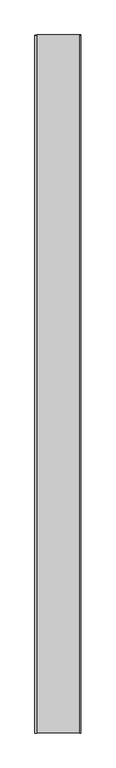
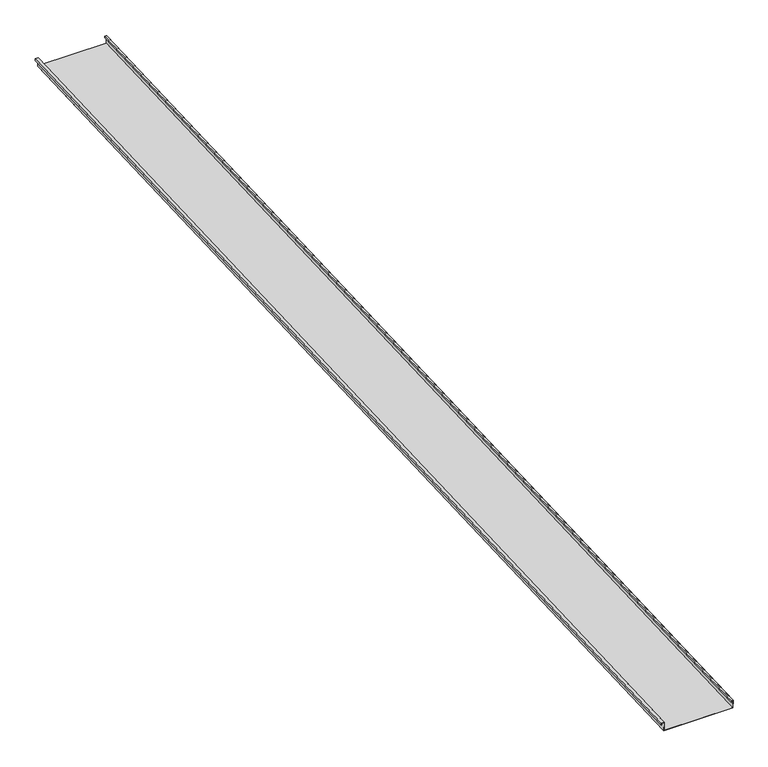
"""IFC4 building model written with IfcOpenShell, lengths in millimetres: proxy geometry, Generic Models 2:Generic Models 2:310765:Generic Models 2:310765 : Generic Models 2:Generic Models 2:310765:128 : Generic Models 2:Generic Models 2:310765:Generic Models 2:310765 : Generic Models 2:Generic Models 2:310765:300385."""

from ifc_helpers import new_model, si_unit, frame, origin, place, context, project, spatial, polyline, outline, extrude, source, transform, mapped, element, save


def generic_models_a78d9589(model_context):
    return source(origin(), model_context, "Body", "SweptSolid", [
        extrude(outline(polyline([(1.5875, 0.0), (1.5875, 50.8), (407.9875, 50.8), (407.9875, 1.5875), (396.875, 1.5875), (396.875, 11.1125), (398.4625, 11.1125), (398.4625, 3.175), (406.4, 3.175), (406.4, 49.2125), (3.175, 49.2125), (3.175, -1.5874999), (-14.2875, -1.5874999), (-14.2875, 9.525), (-12.7, 9.525), (-12.7, 0.0), (1.5875, 0.0)])), frame((662167.0096405, -581354.4345603, 3902.6697972), z_axis=(0.0, 0.9991330730923568, 0.041630544712067834), x_axis=(1.0, 0.0, 0.0)), (0.0, 0.0, 1.0), 6400.8),
    ])


if __name__ == "__main__":
    model = new_model("IFC4")
    model_context = context("Model", 3, world=origin())
    ifc_project = project(units=[si_unit("LENGTHUNIT", "METRE", prefix="MILLI")], contexts=[model_context])
    site = spatial("IfcSite", under=ifc_project)
    building = spatial("IfcBuilding", under=site)
    placement = place(None, origin())
    generic_models_shape = generic_models_a78d9589(model_context)
    element("IfcBuildingElementProxy", 1, Name="Generic Models 2:Generic Models 2:310765:Generic Models 2:310765 : Generic Models 2:Generic Models 2:310765:128 : Generic Models 2:Generic Models 2:310765:Generic Models 2:310765 : Generic Models 2:Generic Models 2:310765:300385", ObjectType="Generic Models 2:Generic Models 2:310765:Generic Models 2:310765 : Generic Models 2:Generic Models 2:310765:128 : Generic Models 2:Generic Models 2:310765:Generic Models 2:310765 : Generic Models 2:Generic Models 2:310765:300385", at=placement, inside=building, context=model_context, shape_type="MappedRepresentation", body=[
        mapped(generic_models_shape, transform((0.0, 0.0, 0.0), x_axis=(1.0, 0.0, 0.0), y_axis=(0.0, 1.0, 0.0), z_axis=(0.0, 0.0, 1.0))),
    ])
    save(model, "model.ifc")

# Revit data of these elements
# Type "Generic Models 2:Generic Models 2:310765:Generic Models 2:310765 : Generic Models 2:Generic Models 2:310765:128 : Generic Models 2:Generic Models 2:310765:Generic Models 2:310765 : Generic Models 2:Generic Models 2:310765:300385"
#   NameOverride = "Generic Models 2:Generic Models 2:310765:Generic Models 2:310765 : Generic Models 2:Generic Models 2:310765:300385"
#   ObjectTypeOverride = "Generic Models 2:310765 : Generic Models 2:Generic Models 2:310765"
#   Reference = "Generic Models 2"
#   Tag = "300385"
# Element 1 (IfcBuildingElementProxy, "Generic Models 2:Generic Models 2:310765:Generic Models 2:310765 : Generic Models 2:Generic Models 2:310765:128 : Generic Models 2:Generic Models 2:310765:Generic Models 2:310765 : Generic Models 2:Generic Models 2:310765:300385")
#   Materials on its faces: "THERMAL BROKEN ALUMINUM STOREFRONT FOR POLYCARBONATE"
# Materials
#   "THERMAL BROKEN ALUMINUM STOREFRONT FOR POLYCARBONATE": class "Unassigned", colour RGB 244 244 244, transparency 0, Keynote = "M07611300.01", Cost = 0
